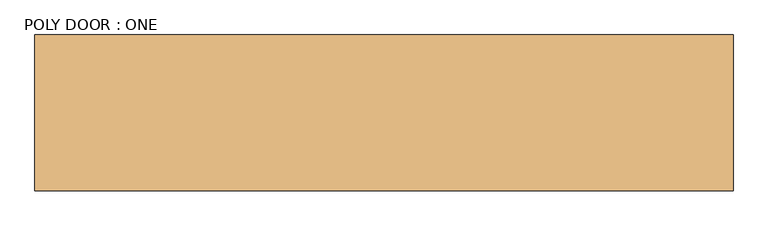
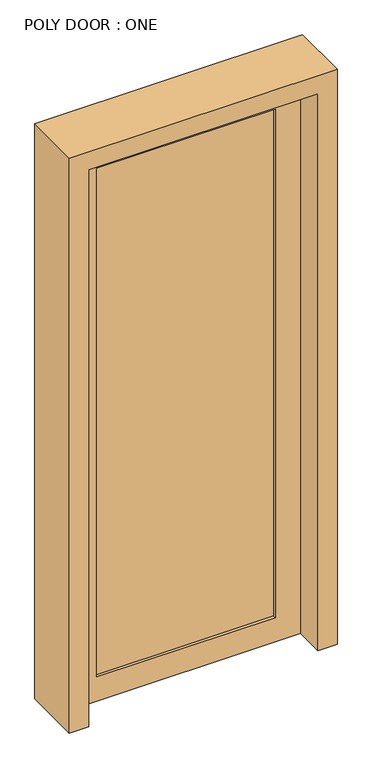
"""IFC4 building model written with IfcOpenShell, lengths in millimetres: door geometry, POLY DOOR : ONE."""

from ifc_helpers import new_model, si_unit, frame, origin, place, context, project, spatial, polyline, outline, extrude, source, transform, mapped, element, save


def poly_door_one_7be98fc3(model_context):
    return source(origin(), model_context, "Body", "SweptSolid", [
        extrude(outline(polyline([(355.6, 25.4), (355.6, 12.7), (-355.6, 12.7), (-355.6, 25.4), (355.6, 25.4)])), frame((0.0, 0.0, 101.6), z_axis=(0.0, 0.0, 1.0), x_axis=(1.0, 0.0, 0.0)), (0.0, 0.0, 1.0), 2139.95),
        extrude(outline(polyline([(2343.15, 457.2), (2343.15, -457.2), (0.0, -457.2), (0.0, 457.2), (2343.15, 457.2)]), holes=[polyline([(2241.55, 355.6), (101.6, 355.6), (101.6, -355.6), (2241.55, -355.6), (2241.55, 355.6)])]), frame((0.0, 0.0, 0.0), z_axis=(0.0, 1.0, 0.0), x_axis=(0.0, 0.0, 1.0)), (0.0, 0.0, 1.0), 50.8),
        extrude(outline(polyline([(2419.35, -533.4), (0.0, -533.4), (0.0, -457.2), (2343.15, -457.2), (2343.15, 457.2), (0.0, 457.2), (0.0, 533.4), (2419.35, 533.4), (2419.35, -533.4)])), frame((0.0, -119.0625, 0.0), z_axis=(0.0, 1.0, 0.0), x_axis=(0.0, 0.0, 1.0)), (0.0, 0.0, 1.0), 238.125),
    ])


if __name__ == "__main__":
    model = new_model("IFC4")
    model_context = context("Model", 3, world=origin())
    ifc_project = project(units=[si_unit("LENGTHUNIT", "METRE", prefix="MILLI")], contexts=[model_context])
    site = spatial("IfcSite", under=ifc_project)
    building = spatial("IfcBuilding", under=site)
    placement = place(None, origin())
    poly_door_one_shape = poly_door_one_7be98fc3(model_context)
    element("IfcDoor", 1, ObjectType="POLY DOOR : ONE", at=placement, inside=building, context=model_context, shape_type="MappedRepresentation", body=[
        mapped(poly_door_one_shape, transform((0.0, 0.0, 0.0), x_axis=(1.0, 0.0, 0.0), y_axis=(0.0, 1.0, 0.0), z_axis=(0.0, 0.0, 1.0))),
    ])
    save(model, "model.ifc")

# Revit data of these elements
# Type "POLY DOOR : ONE"
#   Type Mark = "53"
#   Assembly Code = "C1020"
#   Analytic Construction = "<None>"
#   Thickness = 0' - 2"
#   Glass Inset = 0' - 4"
#   Height = 7' - 8 1/4"
#   Trim Projection Ext = 0' - 1"
#   Trim Projection Int = 0' - 1"
#   Trim Width = 0' - 3"
#   Width = 3' - 0"
#   WINDOW = yes
#   Glass Material = ALUM. STOREFRONT W/ INSULATED GLAZING
#   Door Material = Aluminum
#   Frame Material = Aluminum
#   Function = (empty or 0)
#   Wall Closure = (empty or 0)
# Element 1 (IfcDoor, "POLY DOOR : ONE")
#   Materials on its faces: "Aluminum", "ALUM. STOREFRONT W/ INSULATED GLAZING"
# Materials
#   "ALUM. STOREFRONT W/ INSULATED GLAZING": class "Glass", colour RGB 196 205 210, transparency 0.85, Description = "Soda Lime Glass", Cost = 0
#   "Aluminum": class "Metal", colour RGB 244 244 244, transparency 0, Description = "Aluminum 6061", Cost = 0
